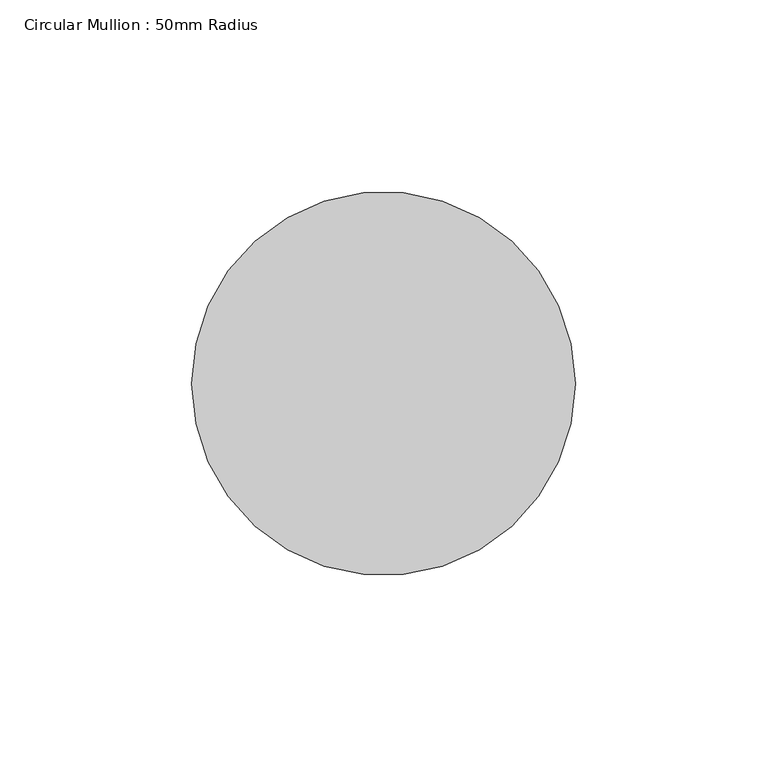
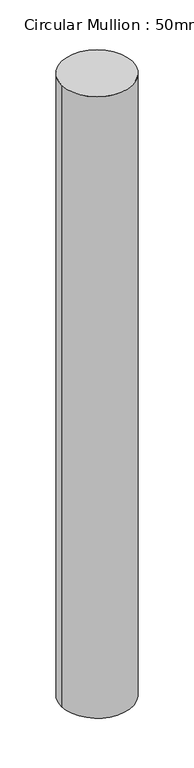
"""IFC4 building model written with IfcOpenShell, lengths in millimetres: member geometry, Circular Mullion : 50mm Radius."""

from ifc_helpers import new_model, si_unit, point, frame, origin, origin_2d, place, context, project, spatial, circle_curve, trimmed, segment, composite_curve, outline, extrude, source, transform, mapped, element, save


def circular_mullion_50mm_radius_7ab57a74(model_context):
    return source(origin(), model_context, "Body", "SweptSolid", [
        extrude(outline(composite_curve([segment(trimmed(circle_curve(origin_2d(), 50.0), [point((50.0, 0.0))], [point((-50.0, 0.0))], False, "CARTESIAN"), True, "CONTINUOUS"), segment(trimmed(circle_curve(origin_2d(), 50.0), [point((-50.0, 0.0))], [point((50.0, 0.0))], False, "CARTESIAN"), True, "CONTINUOUS")], self_intersect=False)), frame((0.0, 0.0, -923.2904119), z_axis=(0.0, 0.0, 1.0), x_axis=(1.0, 0.0, 0.0)), (0.0, 0.0, 1.0), 923.2904119),
    ])


if __name__ == "__main__":
    model = new_model("IFC4")
    model_context = context("Model", 3, world=origin())
    ifc_project = project(units=[si_unit("LENGTHUNIT", "METRE", prefix="MILLI")], contexts=[model_context])
    site = spatial("IfcSite", under=ifc_project)
    building = spatial("IfcBuilding", under=site)
    placement = place(None, origin())
    circular_mullion_50mm_radius_shape = circular_mullion_50mm_radius_7ab57a74(model_context)
    element("IfcMember", 1, ObjectType="Circular Mullion : 50mm Radius", at=placement, inside=building, context=model_context, shape_type="MappedRepresentation", body=[
        mapped(circular_mullion_50mm_radius_shape, transform((0.0, 0.0, 0.0), x_axis=(1.0, 0.0, 0.0), y_axis=(0.0, 1.0, 0.0), z_axis=(0.0, 0.0, 1.0))),
    ])
    save(model, "model.ifc")

# Revit data of these elements
# Type "Circular Mullion : 50mm Radius"
#   built-in parameter 1007350 = 0.164042 (stored number, unit not read)
# Element 1 (IfcMember, "Circular Mullion : 50mm Radius")
#   Materials on its faces: "Aluminium"
# Materials
#   "Aluminium": class "Metal", colour RGB 247 247 247, transparency 0, Description = "Aluminium 6061", Cost = 0
